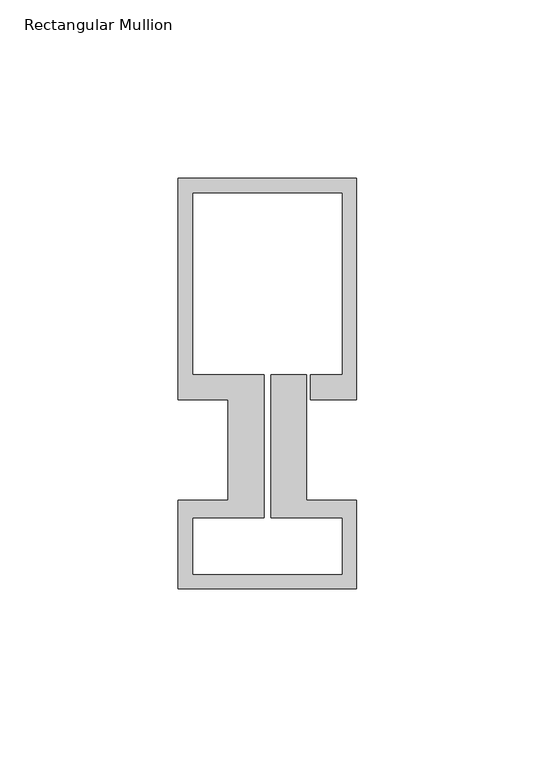
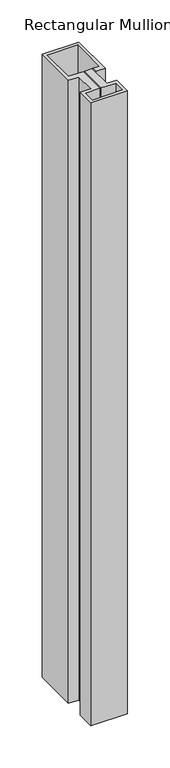
"""IFC4 building model written with IfcOpenShell, lengths in millimetres: member geometry, Rectangular Mullion : Schueco_FWS-50-HI_Tran_CovCap-20mm_Tran-55mm."""

from ifc_helpers import new_model, si_unit, frame, origin, place, context, project, spatial, polyline, outline, extrude, source, transform, mapped, element, save


def rectangular_mullion_e28d13dc(model_context):
    return source(origin(), model_context, "Body", "SweptSolid", [
        extrude(outline(polyline([(-50.0, 90.0), (0.0, 90.0), (0.0, 28.0), (-13.0, 28.0), (-13.0, 35.0), (-4.0, 35.0), (-4.0, 86.0), (-46.0, 86.0), (-46.0, 35.0), (-26.0, 35.0), (-26.0, -5.0), (-46.0, -5.0), (-46.0, -21.0), (-4.0, -21.0), (-4.0, -5.0), (-24.0, -5.0), (-24.0, 35.0), (-14.0, 35.0), (-14.0, -0.1), (0.0, -0.1), (0.0, -25.0), (-50.0, -25.0), (-50.0, -0.1), (-36.0, -0.1), (-36.0, 28.0), (-50.0, 28.0), (-50.0, 90.0)])), frame((0.0, 0.0, -900.0), z_axis=(0.0, 0.0, 1.0), x_axis=(1.0, 0.0, 0.0)), (0.0, 0.0, 1.0), 900.0),
    ])


if __name__ == "__main__":
    model = new_model("IFC4")
    model_context = context("Model", 3, world=origin())
    ifc_project = project(units=[si_unit("LENGTHUNIT", "METRE", prefix="MILLI")], contexts=[model_context])
    site = spatial("IfcSite", under=ifc_project)
    building = spatial("IfcBuilding", under=site)
    placement = place(None, origin())
    rectangular_mullion_shape = rectangular_mullion_e28d13dc(model_context)
    element("IfcMember", 1, ObjectType="Rectangular Mullion : Schueco_FWS-50-HI_Tran_CovCap-20mm_Tran-55mm", at=placement, inside=building, context=model_context, shape_type="MappedRepresentation", body=[
        mapped(rectangular_mullion_shape, transform((0.0, 0.0, 0.0), x_axis=(1.0, 0.0, 0.0), y_axis=(0.0, 1.0, 0.0), z_axis=(0.0, 0.0, 1.0))),
    ])
    save(model, "model.ifc")

# Revit data of these elements
# Type "Rectangular Mullion : Schueco_FWS-50-HI_Tran_CovCap-20mm_Tran-55mm"
#   Model = "FWS 50.HI"
#   Manufacturer = "Schueco International KG"
#   Type Comments = "Transom"
#   Schueco thermal insulation standard = "Highly thermally insulated"
#   Burglar resistance = "RC 3"
#   Thermal insulation = "to 0.90 W/(m²K)"
#   built-in parameter 1007322 = 0.377297 (stored number, unit not read)
#   built-in parameter 1007321 = 0.0360892 (stored number, unit not read)
#   built-in parameter 1007320 = 0.0360892 (stored number, unit not read)
# Element 1 (IfcMember, "Rectangular Mullion : Schueco_FWS-50-HI_Tran_CovCap-20mm_Tran-55mm")
#   Materials on its faces: "Alu"
# Materials
#   "Alu": class "Glas", colour RGB 140 140 140, transparency 0
